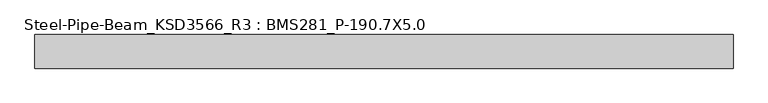
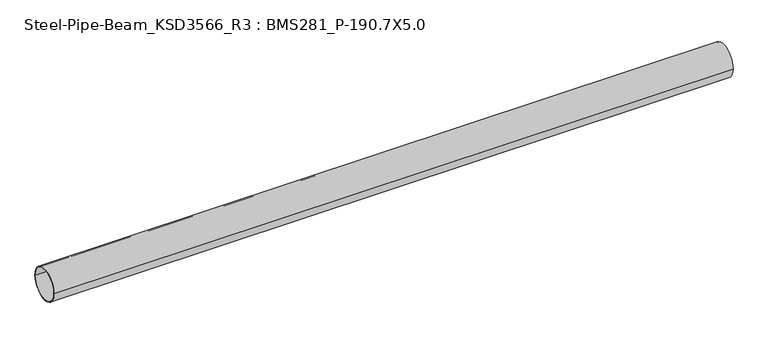
"""IFC4 building model written with IfcOpenShell, lengths in millimetres: member geometry, Steel-Pipe-Beam_KSD3566_R3 : BMS281_P-190.7X5.0."""

from ifc_helpers import new_model, si_unit, point, frame, origin, origin_2d, place, context, project, spatial, circle_curve, trimmed, segment, composite_curve, outline, extrude, source, transform, mapped, element, save


def steel_pipe_beam_ksd3566_r3_bms281_p_190_7x5_0_5b1fd4fb(model_context):
    return source(origin(), model_context, "Body", "SweptSolid", [
        extrude(outline(composite_curve([segment(trimmed(circle_curve(origin_2d(), 95.35), [point((-95.35, 0.0))], [point((95.35, 0.0))], False, "CARTESIAN"), True, "CONTINUOUS"), segment(trimmed(circle_curve(origin_2d(), 95.35), [point((95.35, 0.0))], [point((-95.35, 0.0))], False, "CARTESIAN"), True, "CONTINUOUS")], self_intersect=False), holes=[composite_curve([segment(trimmed(circle_curve(origin_2d(), 90.35), [point((90.35, 0.0))], [point((-90.35, 0.0))], True, "CARTESIAN"), True, "CONTINUOUS"), segment(trimmed(circle_curve(origin_2d(), 90.35), [point((-90.35, 0.0))], [point((90.35, 0.0))], True, "CARTESIAN"), True, "CONTINUOUS")], self_intersect=False)]), frame((-1979.4197168, 0.0, 0.0), z_axis=(1.0, 0.0, 0.0), x_axis=(0.0, 1.0, 0.0)), (0.0, 0.0, 1.0), 3955.0697889),
    ])


if __name__ == "__main__":
    model = new_model("IFC4")
    model_context = context("Model", 3, world=origin())
    ifc_project = project(units=[si_unit("LENGTHUNIT", "METRE", prefix="MILLI")], contexts=[model_context])
    site = spatial("IfcSite", under=ifc_project)
    building = spatial("IfcBuilding", under=site)
    placement = place(None, origin())
    steel_pipe_beam_ksd3566_r3_bms281_p_190_7x5_0_shape = steel_pipe_beam_ksd3566_r3_bms281_p_190_7x5_0_5b1fd4fb(model_context)
    element("IfcMember", 1, ObjectType="Steel-Pipe-Beam_KSD3566_R3 : BMS281_P-190.7X5.0", at=placement, inside=building, context=model_context, shape_type="MappedRepresentation", body=[
        mapped(steel_pipe_beam_ksd3566_r3_bms281_p_190_7x5_0_shape, transform((0.0, 0.0, 0.0), x_axis=(1.0, 0.0, 0.0), y_axis=(0.0, 1.0, 0.0), z_axis=(0.0, 0.0, 1.0))),
    ])
    save(model, "model.ifc")

# Revit data of these elements
# Type "Steel-Pipe-Beam_KSD3566_R3 : BMS281_P-190.7X5.0"
#   Keynote = "P-190.7X5.0"
#   SteelWeight = "Light"
#   t = 0.0050 m
#   Surface Area = 0.599102 m²/m
#   Section Area = 29.1697 cm²
#   Mass per Unit Length = 22.8982 kg/m
#   Length [instance default] = 1.5000 m
#   D = 0.1907 m
#   hec_material4 [instance default] = none
#   hec_material3 [instance default] = none
#   hec_material2 [instance default] = none
#   hec_material1 [instance default] = none
#   Structural Material [instance default] = Steel, 45-345
#   Assembly Code = ""
# Element 1 (IfcMember, "Steel-Pipe-Beam_KSD3566_R3 : BMS281_P-190.7X5.0")
#   Structural Material = none
# Materials
#   "Steel, 45-345": class "Metal", colour RGB 189 187 185, transparency 0, Description = "Steel 345 MPa", Cost = 0
